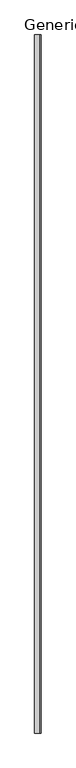
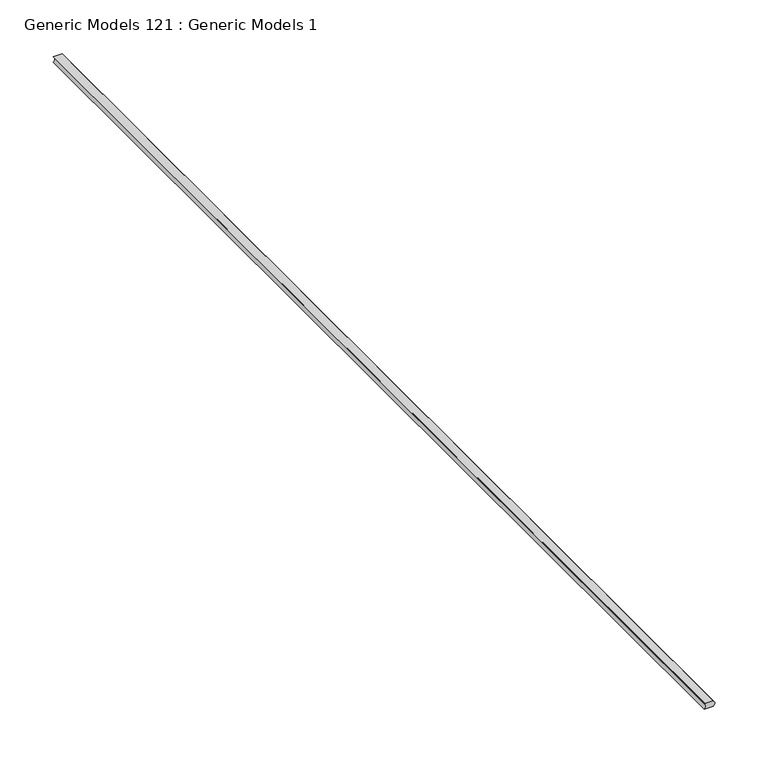
"""IFC4 building model written with IfcOpenShell, lengths in millimetres: proxy geometry, Generic Models 121 : Generic Models 1."""

import ifcopenshell
import ifcopenshell.guid

model = None  # the IFC model being written
_history = None  # IfcOwnerHistory: only IFC2X3 demands one
_inside = {}  # id of a spatial element -> (the spatial element, [elements in it])
_under = {}  # id of a project, library or spatial element -> (it, [spatial elements below it])
_declared = {}  # id of a project -> (the project, [libraries it declares])
_typed = {}  # id of a type object -> (the type object, [elements of that type])
_made_of = {}  # id of a material, layer set ... -> (it, [elements and type objects made of it])


def new_model(schema):
    """Start an empty IFC model of exactly this schema.

    Asked for "IFC4X3", IfcOpenShell would pick the latest addendum, in which some entities
    have other attributes; the version numbers below select the first issue.
    IFC2X3 requires an IfcOwnerHistory on every rooted entity: one is made here for all.
    """
    global model, _history
    if schema == "IFC4X3":
        model = ifcopenshell.file(schema_version=(4, 3, 0, 0))
    else:
        model = ifcopenshell.file(schema=schema)
    _inside.clear()
    _under.clear()
    _declared.clear()
    _typed.clear()
    _made_of.clear()
    _history = None
    if model.schema == "IFC2X3":
        org = make("IfcOrganization", Name="unknown")
        user = make(
            "IfcPersonAndOrganization",
            ThePerson=make("IfcPerson", FamilyName="unknown"),
            TheOrganization=org,
        )
        app = make(
            "IfcApplication",
            ApplicationDeveloper=org,
            Version="unknown",
            ApplicationFullName="unknown",
            ApplicationIdentifier="unknown",
        )
        _history = make(
            "IfcOwnerHistory",
            OwningUser=user,
            OwningApplication=app,
            ChangeAction="ADDED",
            CreationDate=0,
        )
    return model


def make(cls, **values):
    """One entity of the class cls with the attributes given. An attribute that is None is left unset."""
    return model.create_entity(
        cls, **{name: value for name, value in values.items() if value is not None}
    )


def rooted(cls, **values):
    """An entity with a GlobalId (a new one), such as an element, a storey or a relation."""
    return make(cls, GlobalId=ifcopenshell.guid.new(), OwnerHistory=_history, **values)


def si_unit(unit_type, name, prefix=None):
    """IfcSIUnit, for example si_unit("LENGTHUNIT", "METRE", prefix="MILLI")."""
    return make("IfcSIUnit", UnitType=unit_type, Prefix=prefix, Name=name)


def assignment(units):
    """IfcUnitAssignment: the units of a project."""
    return None if units is None else make("IfcUnitAssignment", Units=units)


def point(xyz):
    """IfcCartesianPoint."""
    return None if xyz is None else make("IfcCartesianPoint", Coordinates=xyz)


def direction(xyz):
    """IfcDirection."""
    return None if xyz is None else make("IfcDirection", DirectionRatios=xyz)


def frame(location, z_axis=None, x_axis=None):
    """IfcAxis2Placement3D, a coordinate frame: its origin and axes. An axis left out is left unset."""
    return make(
        "IfcAxis2Placement3D",
        Location=point(location),
        Axis=direction(z_axis),
        RefDirection=direction(x_axis),
    )


def frame_2d(location, x_axis=None):
    """IfcAxis2Placement2D, a coordinate frame in the plane: its origin and x axis."""
    return make(
        "IfcAxis2Placement2D", Location=point(location), RefDirection=direction(x_axis)
    )


def origin():
    """The frame at (0, 0, 0) with its axes left unset."""
    return frame((0.0, 0.0, 0.0))


def place(relative_to, where):
    """IfcLocalPlacement: puts the frame where relative to a parent placement (None: the world)."""
    return make(
        "IfcLocalPlacement", PlacementRelTo=relative_to, RelativePlacement=where
    )


def context(
    kind, dimensions, precision=None, world=None, true_north=None, identifier=None
):
    """IfcGeometricRepresentationContext, for example the 3D "Model" context."""
    return make(
        "IfcGeometricRepresentationContext",
        ContextIdentifier=identifier,
        ContextType=kind,
        CoordinateSpaceDimension=dimensions,
        Precision=precision,
        WorldCoordinateSystem=world,
        TrueNorth=true_north,
    )


def project(units=None, contexts=None):
    """IfcProject with its units and contexts."""
    return rooted(
        "IfcProject",
        Name="project",
        RepresentationContexts=contexts,
        UnitsInContext=assignment(units),
    )


def spatial(cls, under=None, at=None, **own):
    """A site, building, storey or space (cls), placed at a placement, below another one or the project."""
    s = rooted(cls, ObjectPlacement=at, **own)
    if under is not None:
        _under.setdefault(under.id(), (under, []))[1].append(s)
    return s


def polyline(points):
    """IfcPolyline through the points."""
    return make("IfcPolyline", Points=[point(p) for p in points])


def circle_curve(where, radius):
    """IfcCircle in the frame where."""
    return make("IfcCircle", Position=where, Radius=radius)


def trimmed(basis, trim1, trim2, sense, master):
    """IfcTrimmedCurve: the piece of a basis curve between two trims."""
    return make(
        "IfcTrimmedCurve",
        BasisCurve=basis,
        Trim1=trim1,
        Trim2=trim2,
        SenseAgreement=sense,
        MasterRepresentation=master,
    )


def segment(curve, same_sense, transition):
    """IfcCompositeCurveSegment."""
    return make(
        "IfcCompositeCurveSegment",
        Transition=transition,
        SameSense=same_sense,
        ParentCurve=curve,
    )


def composite_curve(segments, self_intersect=None):
    """IfcCompositeCurve: segments joined end to end."""
    return make("IfcCompositeCurve", Segments=segments, SelfIntersect=self_intersect)


def outline(outer, holes=None, kind="AREA"):
    """IfcArbitraryClosedProfileDef: a profile drawn as a closed curve; with holes, ...WithVoids."""
    if holes is None:
        return make("IfcArbitraryClosedProfileDef", ProfileType=kind, OuterCurve=outer)
    return make(
        "IfcArbitraryProfileDefWithVoids",
        ProfileType=kind,
        OuterCurve=outer,
        InnerCurves=holes,
    )


def extrude(swept, where, along, depth):
    """IfcExtrudedAreaSolid: the profile swept, set in the frame where, extruded along a direction by depth."""
    return make(
        "IfcExtrudedAreaSolid",
        SweptArea=swept,
        Position=where,
        ExtrudedDirection=direction(along),
        Depth=depth,
    )


def shape(context_of_items, identifier, shape_type, items):
    """IfcShapeRepresentation: the items that make up one representation, for example the "Body"."""
    return make(
        "IfcShapeRepresentation",
        ContextOfItems=context_of_items,
        RepresentationIdentifier=identifier,
        RepresentationType=shape_type,
        Items=items,
    )


def source(mapping_origin, context_of_items, identifier, shape_type, items):
    """IfcRepresentationMap: a shape defined once, which mapped items show again and again."""
    return make(
        "IfcRepresentationMap",
        MappingOrigin=mapping_origin,
        MappedRepresentation=shape(context_of_items, identifier, shape_type, items),
    )


def transform(
    local_origin,
    x_axis=None,
    y_axis=None,
    z_axis=None,
    scale=None,
    scale2=None,
    scale3=None,
    uniform=True,
):
    """IfcCartesianTransformationOperator3D, or its non-uniform kind. x_axis, y_axis, z_axis: its Axis1, 2, 3."""
    if uniform:
        return make(
            "IfcCartesianTransformationOperator3D",
            Axis1=direction(x_axis),
            Axis2=direction(y_axis),
            LocalOrigin=point(local_origin),
            Scale=scale,
            Axis3=direction(z_axis),
        )
    return make(
        "IfcCartesianTransformationOperator3DnonUniform",
        Axis1=direction(x_axis),
        Axis2=direction(y_axis),
        LocalOrigin=point(local_origin),
        Scale=scale,
        Axis3=direction(z_axis),
        Scale2=scale2,
        Scale3=scale3,
    )


def mapped(mapping_source, mapping_target):
    """IfcMappedItem: shows the shape of a source again, moved by a transform."""
    return make(
        "IfcMappedItem", MappingSource=mapping_source, MappingTarget=mapping_target
    )


def made_of(thing, what):
    """Note that an element or type object is made of a material, layer set ...; save() writes the relation."""
    if what is not None:
        _made_of.setdefault(what.id(), (what, []))[1].append(thing)
    return thing


def element(
    cls,
    number,
    at=None,
    inside=None,
    cuts=None,
    type_object=None,
    material=None,
    context=None,
    identifier="Body",
    shape_type=None,
    held_by="IfcProductDefinitionShape",
    body=None,
    shapes=None,
    **own,
):
    """One element of the class cls, such as IfcWall. Its Tag is "e" and its number.

    at: its placement. inside: the storey or other place that contains it. cuts: it is an
    opening in that element (IfcRelVoidsElement). A single representation is given by context,
    identifier, shape_type and body (its items); several are given by shapes. held_by: the class
    of the entity that holds the representations. save() writes the other relations.
    """
    e = rooted(cls, Tag="e%d" % number, ObjectPlacement=at, **own)
    if body is not None:
        shapes = [shape(context, identifier, shape_type, body)]
    if shapes is not None:
        e.Representation = make(held_by, Representations=shapes)
    if inside is not None:
        _inside.setdefault(inside.id(), (inside, []))[1].append(e)
    if cuts is not None:
        rooted(
            "IfcRelVoidsElement", RelatingBuildingElement=cuts, RelatedOpeningElement=e
        )
    if type_object is not None:
        _typed.setdefault(type_object.id(), (type_object, []))[1].append(e)
    return made_of(e, material)


def aggregate(whole, parts):
    """IfcRelAggregates: a whole, such as a stair, and the parts it consists of."""
    return rooted("IfcRelAggregates", RelatingObject=whole, RelatedObjects=parts)


def save(model, path):
    """Write the relations noted so far, then the file.

    IfcRelAggregates (storeys below a building ...), IfcRelContainedInSpatialStructure (elements
    in a storey), IfcRelDefinesByType, IfcRelAssociatesMaterial and IfcRelDeclares: one each for
    every whole, place, type object, material and project.
    """
    for whole, parts in _under.values():
        aggregate(whole, parts)
    for where, things in _inside.values():
        rooted(
            "IfcRelContainedInSpatialStructure",
            RelatedElements=things,
            RelatingStructure=where,
        )
    for kind, things in _typed.values():
        rooted("IfcRelDefinesByType", RelatedObjects=things, RelatingType=kind)
    for what, things in _made_of.values():
        rooted("IfcRelAssociatesMaterial", RelatedObjects=things, RelatingMaterial=what)
    for by, libraries in _declared.values():
        rooted("IfcRelDeclares", RelatingContext=by, RelatedDefinitions=libraries)
    model.write(path)


def generic_models_121_generic_models_1_de47f0a2(model_context):
    return source(origin(), model_context, "Body", "SweptSolid", [
        extrude(outline(composite_curve([segment(polyline([(0.0, 48456.85), (0.0, 48466.375)]), True, "CONTINUOUS"), segment(trimmed(circle_curve(frame_2d((3.175, 48463.4602595)), 4.3100275), [point((0.0, 48466.375))], [point((6.35, 48466.375))], False, "CARTESIAN"), True, "CONTINUOUS"), segment(polyline([(6.35, 48466.375), (6.35, 48456.85)]), True, "CONTINUOUS"), segment(trimmed(circle_curve(frame_2d((3.175, 48453.9352595)), 4.3100275), [point((6.35, 48456.85))], [point((0.0, 48456.85))], True, "CARTESIAN"), True, "CONTINUOUS")], self_intersect=False)), frame((0.0, 0.0, 0.0), z_axis=(0.0, 1.0, 0.0), x_axis=(0.0, 0.0, 1.0)), (0.0, 0.0, 1.0), 1219.2),
    ])


if __name__ == "__main__":
    model = new_model("IFC4")
    model_context = context("Model", 3, world=origin())
    ifc_project = project(units=[si_unit("LENGTHUNIT", "METRE", prefix="MILLI")], contexts=[model_context])
    site = spatial("IfcSite", under=ifc_project)
    building = spatial("IfcBuilding", under=site)
    placement = place(None, origin())
    generic_models_121_generic_models_1_shape = generic_models_121_generic_models_1_de47f0a2(model_context)
    element("IfcBuildingElementProxy", 1, Name="Generic Models 121 : Generic Models 1", ObjectType="Generic Models 121 : Generic Models 1", at=placement, inside=building, context=model_context, shape_type="MappedRepresentation", body=[
        mapped(generic_models_121_generic_models_1_shape, transform((0.0, 0.0, 0.0), x_axis=(1.0, 0.0, 0.0), y_axis=(0.0, 1.0, 0.0), z_axis=(0.0, 0.0, 1.0))),
    ])
    save(model, "model.ifc")

# Revit data of these elements
# Element 1 (IfcBuildingElementProxy, "Generic Models 121 : Generic Models 1")
#   Materials on its faces: "ACOUSTICAL SEALANT"
# Materials
#   "ACOUSTICAL SEALANT": class "Unassigned", colour RGB 120 120 120, transparency 0, Cost = 0
